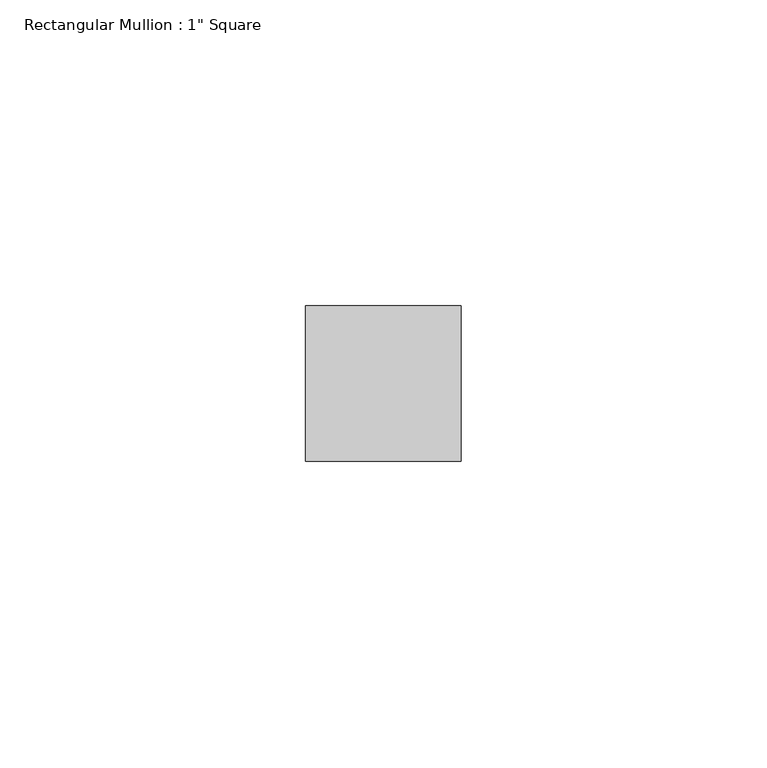
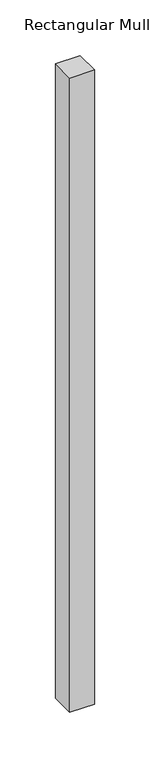
"""IFC4 building model written with IfcOpenShell, lengths in millimetres: member geometry."""

from ifc_helpers import new_model, si_unit, frame, origin, place, context, project, spatial, polyline, outline, extrude, source, transform, mapped, element, save


def member_4863fcab(model_context):
    return source(origin(), model_context, "Body", "SweptSolid", [
        extrude(outline(polyline([(0.0, 12.7), (0.0, -12.7), (-25.4, -12.7), (-25.4, 12.7), (0.0, 12.7)])), frame((0.0, 0.0, -693.7510143), z_axis=(0.0, 0.0, 1.0), x_axis=(1.0, 0.0, 0.0)), (0.0, 0.0, 1.0), 693.7510143),
    ])


if __name__ == "__main__":
    model = new_model("IFC4")
    model_context = context("Model", 3, world=origin())
    ifc_project = project(units=[si_unit("LENGTHUNIT", "METRE", prefix="MILLI")], contexts=[model_context])
    site = spatial("IfcSite", under=ifc_project)
    building = spatial("IfcBuilding", under=site)
    placement = place(None, origin())
    member_shape = member_4863fcab(model_context)
    element("IfcMember", 1, ObjectType="Rectangular Mullion : 1\" Square", at=placement, inside=building, context=model_context, shape_type="MappedRepresentation", body=[
        mapped(member_shape, transform((0.0, 0.0, 0.0), x_axis=(1.0, 0.0, 0.0), y_axis=(0.0, 1.0, 0.0), z_axis=(0.0, 0.0, 1.0))),
    ])
    save(model, "model.ifc")

# Revit data of these elements
# Type "Rectangular Mullion : 1\" Square"
#   built-in parameter 1007304 = 0.0833333 (stored number, unit not read)
#   built-in parameter 1007301 = 0.0416667 (stored number, unit not read)
#   built-in parameter 1007300 = 0.0416667 (stored number, unit not read)
# Element 1 (IfcMember, "Rectangular Mullion : 1\" Square")
#   Materials on its faces: "Metal - Aluminum"
# Materials
#   "Metal - Aluminum": class "Metal", colour RGB 247 247 247, transparency 0
